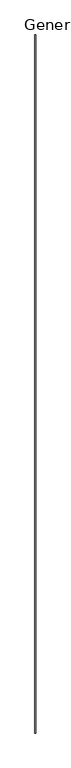
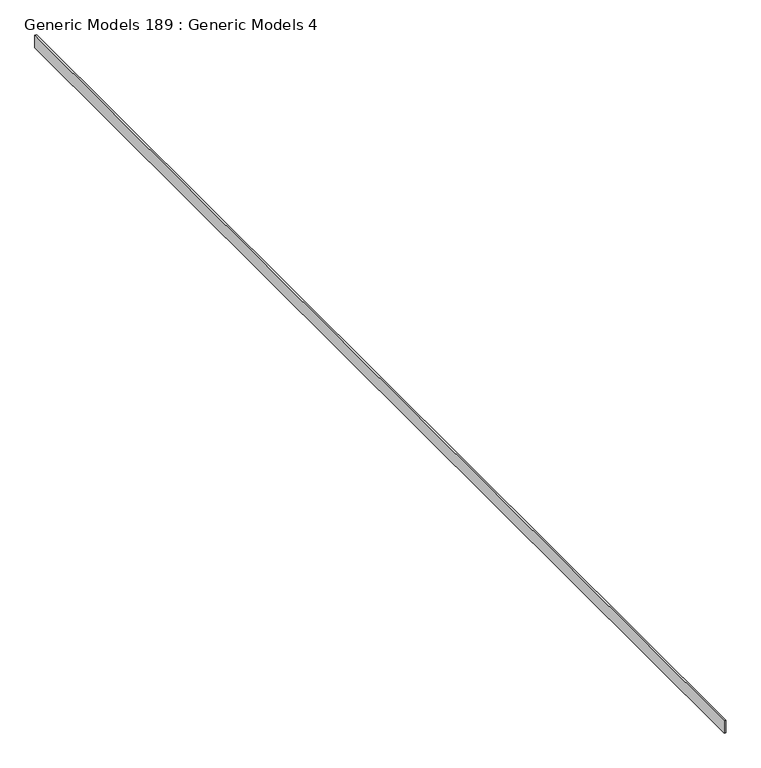
"""IFC4 building model written with IfcOpenShell, lengths in millimetres: proxy geometry, Generic Models 189 : Generic Models 4."""

from ifc_helpers import new_model, si_unit, frame, origin, place, context, project, spatial, polyline, outline, extrude, source, transform, mapped, element, save


def generic_models_189_generic_models_4_522aacdc(model_context):
    return source(origin(), model_context, "Body", "SweptSolid", [
        extrude(outline(polyline([(-5311.9486296, -6864.9230338), (-5330.9986296, -6864.9230338), (-5330.9986296, 7054.2769662), (-5311.9486296, 7054.2769662), (-5311.9486296, -6864.9230338)])), frame((0.0, 0.0, 129255.2221023), z_axis=(0.0, 0.0, 1.0), x_axis=(1.0, 0.0, 0.0)), (0.0, 0.0, 1.0), 154.4259718),
    ])


if __name__ == "__main__":
    model = new_model("IFC4")
    model_context = context("Model", 3, world=origin())
    ifc_project = project(units=[si_unit("LENGTHUNIT", "METRE", prefix="MILLI")], contexts=[model_context])
    site = spatial("IfcSite", under=ifc_project)
    building = spatial("IfcBuilding", under=site)
    placement = place(None, origin())
    generic_models_189_generic_models_4_shape = generic_models_189_generic_models_4_522aacdc(model_context)
    element("IfcBuildingElementProxy", 1, Name="Generic Models 189 : Generic Models 4", ObjectType="Generic Models 189 : Generic Models 4", at=placement, inside=building, context=model_context, shape_type="MappedRepresentation", body=[
        mapped(generic_models_189_generic_models_4_shape, transform((0.0, 0.0, 0.0), x_axis=(1.0, 0.0, 0.0), y_axis=(0.0, 1.0, 0.0), z_axis=(0.0, 0.0, 1.0))),
    ])
    save(model, "model.ifc")

# Revit data of these elements
# Element 1 (IfcBuildingElementProxy, "Generic Models 189 : Generic Models 4")
#   Materials on its faces: "_T&G FIRE RETARDANT WOOD SOFFIT O/ BUILDING PAPER"
# Materials
#   "_T&G FIRE RETARDANT WOOD SOFFIT O/ BUILDING PAPER": class "Generic", colour RGB 177 130 114, transparency 0, Cost = 0
